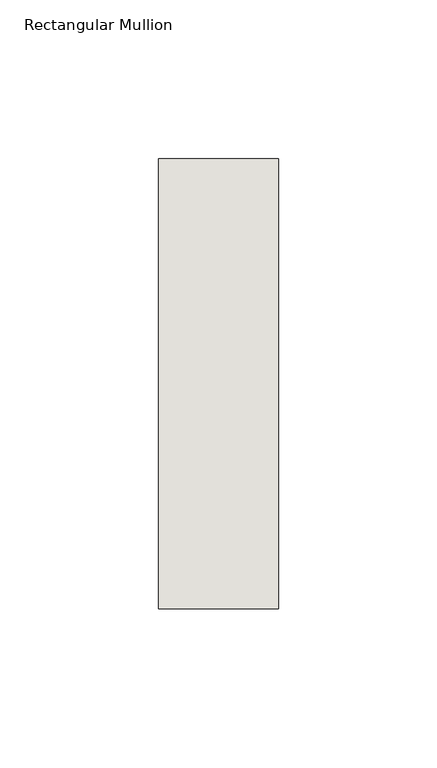
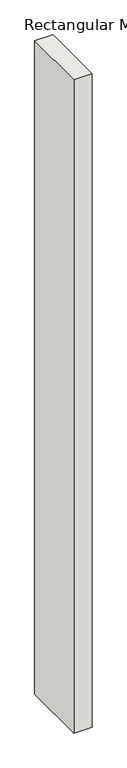
"""IFC4 building model written with IfcOpenShell, lengths in millimetres: wall geometry, Rectangular Mullion : NLRS_21_CWM_hsb-regel 38x142_gen_rsf."""

from ifc_helpers import new_model, si_unit, frame, origin, place, context, project, spatial, polyline, outline, extrude, source, transform, mapped, element, save


def rectangular_mullion_878a7b4c(model_context):
    return source(origin(), model_context, "Body", "SweptSolid", [
        extrude(outline(polyline([(19.0, -71.0), (-19.0, -71.0), (-19.0, 71.0), (19.0, 71.0), (19.0, -71.0)])), frame((0.0, 0.0, -1440.0), z_axis=(0.0, 0.0, 1.0), x_axis=(1.0, 0.0, 0.0)), (0.0, 0.0, 1.0), 1440.0),
    ])


if __name__ == "__main__":
    model = new_model("IFC4")
    model_context = context("Model", 3, world=origin())
    ifc_project = project(units=[si_unit("LENGTHUNIT", "METRE", prefix="MILLI")], contexts=[model_context])
    site = spatial("IfcSite", under=ifc_project)
    building = spatial("IfcBuilding", under=site)
    placement = place(None, origin())
    rectangular_mullion_shape = rectangular_mullion_878a7b4c(model_context)
    element("IfcWall", 1, ObjectType="Rectangular Mullion : NLRS_21_CWM_hsb-regel 38x142_gen_rsf", at=placement, inside=building, context=model_context, shape_type="MappedRepresentation", body=[
        mapped(rectangular_mullion_shape, transform((0.0, 0.0, 0.0), x_axis=(1.0, 0.0, 0.0), y_axis=(0.0, 1.0, 0.0), z_axis=(0.0, 0.0, 1.0))),
    ])
    save(model, "model.ifc")

# Revit data of these elements
# Type "Rectangular Mullion : NLRS_21_CWM_hsb-regel 38x142_gen_rsf"
#   Type IfcGUID = "07M7mRoiH1CR8m_RSKIwpF"
#   Assembly Code = "21.10"
#   IfcExportAs = "IfcWall"
#   built-in parameter 1007322 = 0.465879 (stored number, unit not read)
#   built-in parameter 1007321 = 0.062336 (stored number, unit not read)
#   built-in parameter 1007320 = 0.062336 (stored number, unit not read)
# Element 1 (IfcWall, "Rectangular Mullion : NLRS_21_CWM_hsb-regel 38x142_gen_rsf")
#   Materials on its faces: "NLRS_i2_hout naaldhout vuren_gen_rsf"
# Materials
#   "NLRS_i2_hout naaldhout vuren_gen_rsf": class "I - Hout", colour RGB 234 199 147, transparency 0, Keynote = "i2", Manufacturer = "Revit Standards Foundation", URL = "www.revitstandards.org", Description = "hout vuren", Cost = 0
